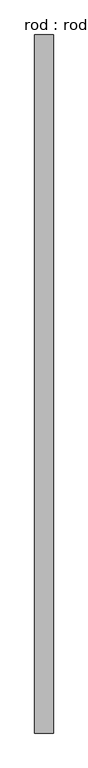
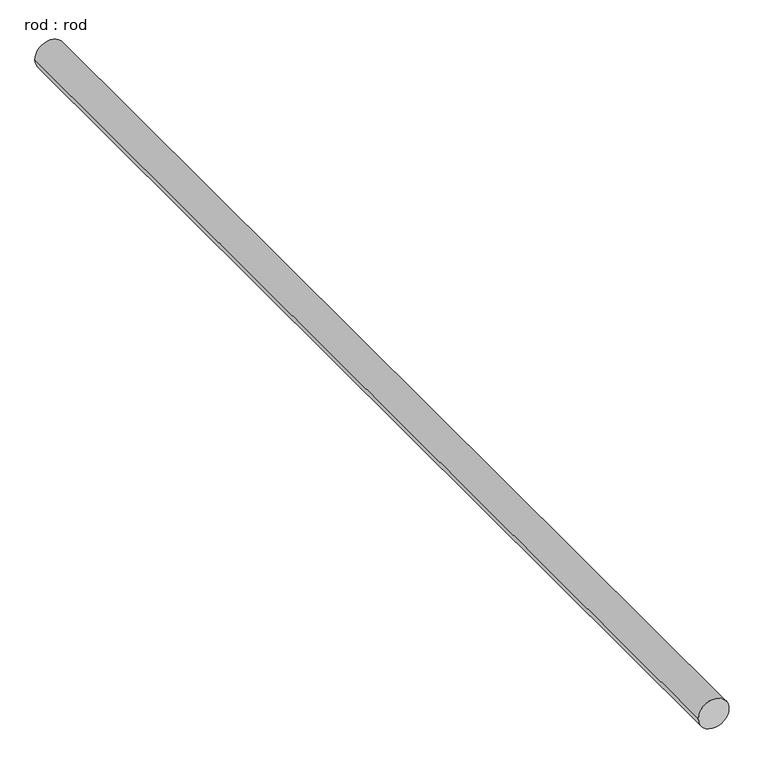
"""IFC4 building model written with IfcOpenShell, lengths in millimetres: proxy geometry, rod : rod."""

from ifc_helpers import new_model, si_unit, point, frame, frame_2d, origin, place, context, project, spatial, circle_curve, trimmed, segment, composite_curve, outline, extrude, source, transform, mapped, element, save


def rod_rod_4bbff020(model_context):
    return source(origin(), model_context, "Body", "SweptSolid", [
        extrude(outline(composite_curve([segment(trimmed(circle_curve(frame_2d((0.0108462, 0.0)), 200.0), [point((0.0108462, 200.0))], [point((0.0108462, -200.0))], False, "CARTESIAN"), True, "CONTINUOUS"), segment(trimmed(circle_curve(frame_2d((0.0108462, 0.0)), 200.0), [point((0.0108462, -200.0))], [point((0.0108462, 200.0))], False, "CARTESIAN"), True, "CONTINUOUS")], self_intersect=False)), frame((0.0, -3407.2713847, 0.0), z_axis=(0.0, 1.0, 0.0), x_axis=(0.0, 0.0, 1.0)), (0.0, 0.0, 1.0), 15000.0),
    ])


if __name__ == "__main__":
    model = new_model("IFC4")
    model_context = context("Model", 3, world=origin())
    ifc_project = project(units=[si_unit("LENGTHUNIT", "METRE", prefix="MILLI")], contexts=[model_context])
    site = spatial("IfcSite", under=ifc_project)
    building = spatial("IfcBuilding", under=site)
    placement = place(None, origin())
    rod_rod_shape = rod_rod_4bbff020(model_context)
    element("IfcBuildingElementProxy", 1, Name="rod : rod", ObjectType="rod : rod", at=placement, inside=building, context=model_context, shape_type="MappedRepresentation", body=[
        mapped(rod_rod_shape, transform((0.0, 0.0, 0.0), x_axis=(1.0, 0.0, 0.0), y_axis=(0.0, 1.0, 0.0), z_axis=(0.0, 0.0, 1.0))),
    ])
    save(model, "model.ifc")

# Revit data of these elements
# Type "rod : rod"
#   Default Elevation = 0
